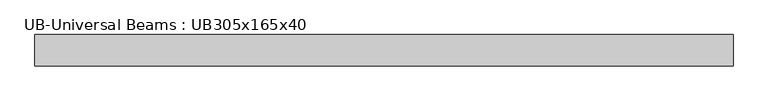
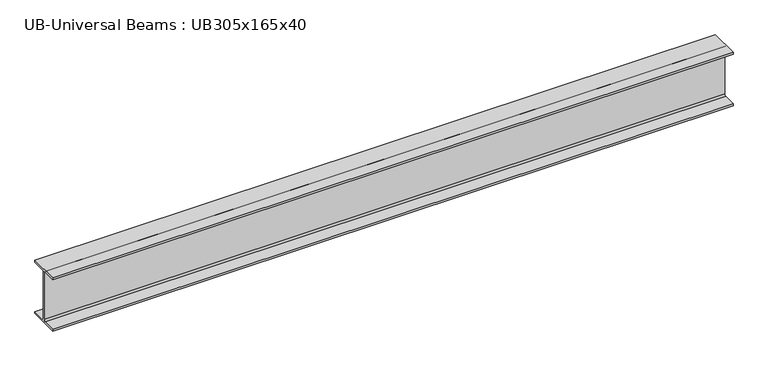
"""IFC4 building model written with IfcOpenShell, lengths in millimetres: beam geometry, UB-Universal Beams : UB305x165x40."""

from ifc_helpers import new_model, si_unit, point, frame, frame_2d, origin, place, context, project, spatial, polyline, circle_curve, trimmed, segment, composite_curve, outline, extrude, source, transform, mapped, element, save


def ub_universal_beams_ub305x165x40_037cda9e(model_context):
    return source(origin(), model_context, "Body", "SweptSolid", [
        extrude(outline(composite_curve([segment(polyline([(82.5, -141.5), (82.5, -151.7), (-82.5, -151.7), (-82.5, -141.5), (-11.9, -141.5)]), True, "CONTINUOUS"), segment(trimmed(circle_curve(frame_2d((-11.9, -132.6)), 8.9), [point((-11.9, -141.5))], [point((-3.0, -132.6))], True, "CARTESIAN"), True, "CONTINUOUS"), segment(polyline([(-3.0, -132.6), (-3.0, 132.6)]), True, "CONTINUOUS"), segment(trimmed(circle_curve(frame_2d((-11.9, 132.6)), 8.9), [point((-3.0, 132.6))], [point((-11.9, 141.5))], True, "CARTESIAN"), True, "CONTINUOUS"), segment(polyline([(-11.9, 141.5), (-82.5, 141.5), (-82.5, 151.7), (82.5, 151.7), (82.5, 141.5), (11.9, 141.5)]), True, "CONTINUOUS"), segment(trimmed(circle_curve(frame_2d((11.9, 132.6)), 8.9), [point((11.9, 141.5))], [point((3.0, 132.6))], True, "CARTESIAN"), True, "CONTINUOUS"), segment(polyline([(3.0, 132.6), (3.0, -132.6)]), True, "CONTINUOUS"), segment(trimmed(circle_curve(frame_2d((11.9, -132.6)), 8.9), [point((3.0, -132.6))], [point((11.9, -141.5))], True, "CARTESIAN"), True, "CONTINUOUS"), segment(polyline([(11.9, -141.5), (82.5, -141.5)]), True, "CONTINUOUS")], self_intersect=False)), frame((-1834.6, 0.0, 0.0), z_axis=(1.0, 0.0, 0.0), x_axis=(0.0, 1.0, 0.0)), (0.0, 0.0, 1.0), 3669.2),
    ])


if __name__ == "__main__":
    model = new_model("IFC4")
    model_context = context("Model", 3, world=origin())
    ifc_project = project(units=[si_unit("LENGTHUNIT", "METRE", prefix="MILLI")], contexts=[model_context])
    site = spatial("IfcSite", under=ifc_project)
    building = spatial("IfcBuilding", under=site)
    placement = place(None, origin())
    ub_universal_beams_ub305x165x40_shape = ub_universal_beams_ub305x165x40_037cda9e(model_context)
    element("IfcBeam", 1, ObjectType="UB-Universal Beams : UB305x165x40", at=placement, inside=building, context=model_context, shape_type="MappedRepresentation", body=[
        mapped(ub_universal_beams_ub305x165x40_shape, transform((0.0, 0.0, 0.0), x_axis=(1.0, 0.0, 0.0), y_axis=(0.0, 1.0, 0.0), z_axis=(0.0, 0.0, 1.0))),
    ])
    save(model, "model.ifc")

# Revit data of these elements
# Type "UB-Universal Beams : UB305x165x40"
#   Section Name Key = "UB305X165X40"
#   Width = 16.5 cm
#   Web Thickness = 0.6 cm
#   Web Fillet = 0.89 cm
#   Warping Constant = 164000.0 cm⁶
#   Torsional Moment of Inertia = 14.70 cm⁴
#   Section Area = 51.3 cm²
#   Plastic Modulus weak axis = 142.0 cm³
#   Plastic Modulus strong axis = 623.0 cm³
#   Nominal Weight = 40.2999 kgf/m
#   Moment of Inertia weak axis = 764.00 cm⁴
#   Moment of Inertia strong axis = 8503.00 cm⁴
#   Height = 30.34 cm
#   Flange Thickness = 1.02 cm
#   Elastic Modulus weak axis = 92.6 cm³
#   Elastic Modulus strong axis = 560.0 cm³
#   Centroid Vertical = 15.17 cm
#   Centroid Horizontal = 8.25 cm
#   Bolt Spacing = 9.0 cm
#   Length [instance default] = 1500 mm
#   Structural Material [instance default] = Metal - Steel 43-275
#   Type Comments = ""
#   Assembly Code = ""
# Element 1 (IfcBeam, "UB-Universal Beams : UB305x165x40")
#   Materials on its faces: "Metal - Steel 43-275"
# Materials
#   "Metal - Steel 43-275": class "Metal", colour RGB 247 247 247, transparency 0, Cost = 0
